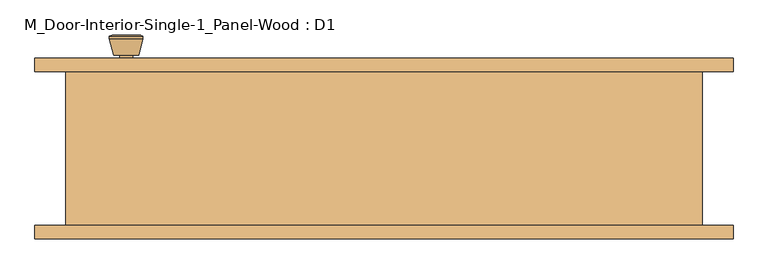
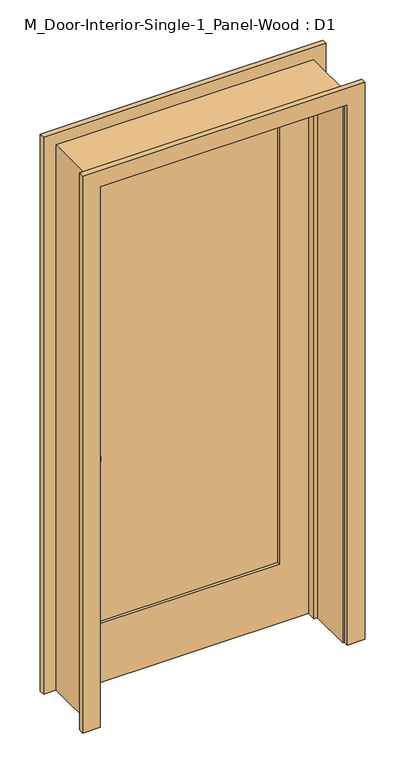
"""IFC4 building model written with IfcOpenShell, lengths in millimetres: door geometry, M_Door-Interior-Single-1_Panel-Wood : D1."""

import ifcopenshell
import ifcopenshell.guid

model = None  # the IFC model being written
_history = None  # IfcOwnerHistory: only IFC2X3 demands one
_inside = {}  # id of a spatial element -> (the spatial element, [elements in it])
_under = {}  # id of a project, library or spatial element -> (it, [spatial elements below it])
_declared = {}  # id of a project -> (the project, [libraries it declares])
_typed = {}  # id of a type object -> (the type object, [elements of that type])
_made_of = {}  # id of a material, layer set ... -> (it, [elements and type objects made of it])


def new_model(schema):
    """Start an empty IFC model of exactly this schema.

    Asked for "IFC4X3", IfcOpenShell would pick the latest addendum, in which some entities
    have other attributes; the version numbers below select the first issue.
    IFC2X3 requires an IfcOwnerHistory on every rooted entity: one is made here for all.
    """
    global model, _history
    if schema == "IFC4X3":
        model = ifcopenshell.file(schema_version=(4, 3, 0, 0))
    else:
        model = ifcopenshell.file(schema=schema)
    _inside.clear()
    _under.clear()
    _declared.clear()
    _typed.clear()
    _made_of.clear()
    _history = None
    if model.schema == "IFC2X3":
        org = make("IfcOrganization", Name="unknown")
        user = make(
            "IfcPersonAndOrganization",
            ThePerson=make("IfcPerson", FamilyName="unknown"),
            TheOrganization=org,
        )
        app = make(
            "IfcApplication",
            ApplicationDeveloper=org,
            Version="unknown",
            ApplicationFullName="unknown",
            ApplicationIdentifier="unknown",
        )
        _history = make(
            "IfcOwnerHistory",
            OwningUser=user,
            OwningApplication=app,
            ChangeAction="ADDED",
            CreationDate=0,
        )
    return model


def make(cls, **values):
    """One entity of the class cls with the attributes given. An attribute that is None is left unset."""
    return model.create_entity(
        cls, **{name: value for name, value in values.items() if value is not None}
    )


def rooted(cls, **values):
    """An entity with a GlobalId (a new one), such as an element, a storey or a relation."""
    return make(cls, GlobalId=ifcopenshell.guid.new(), OwnerHistory=_history, **values)


def si_unit(unit_type, name, prefix=None):
    """IfcSIUnit, for example si_unit("LENGTHUNIT", "METRE", prefix="MILLI")."""
    return make("IfcSIUnit", UnitType=unit_type, Prefix=prefix, Name=name)


def assignment(units):
    """IfcUnitAssignment: the units of a project."""
    return None if units is None else make("IfcUnitAssignment", Units=units)


def point(xyz):
    """IfcCartesianPoint."""
    return None if xyz is None else make("IfcCartesianPoint", Coordinates=xyz)


def direction(xyz):
    """IfcDirection."""
    return None if xyz is None else make("IfcDirection", DirectionRatios=xyz)


def frame(location, z_axis=None, x_axis=None):
    """IfcAxis2Placement3D, a coordinate frame: its origin and axes. An axis left out is left unset."""
    return make(
        "IfcAxis2Placement3D",
        Location=point(location),
        Axis=direction(z_axis),
        RefDirection=direction(x_axis),
    )


def frame_2d(location, x_axis=None):
    """IfcAxis2Placement2D, a coordinate frame in the plane: its origin and x axis."""
    return make(
        "IfcAxis2Placement2D", Location=point(location), RefDirection=direction(x_axis)
    )


def origin():
    """The frame at (0, 0, 0) with its axes left unset."""
    return frame((0.0, 0.0, 0.0))


def place(relative_to, where):
    """IfcLocalPlacement: puts the frame where relative to a parent placement (None: the world)."""
    return make(
        "IfcLocalPlacement", PlacementRelTo=relative_to, RelativePlacement=where
    )


def context(
    kind, dimensions, precision=None, world=None, true_north=None, identifier=None
):
    """IfcGeometricRepresentationContext, for example the 3D "Model" context."""
    return make(
        "IfcGeometricRepresentationContext",
        ContextIdentifier=identifier,
        ContextType=kind,
        CoordinateSpaceDimension=dimensions,
        Precision=precision,
        WorldCoordinateSystem=world,
        TrueNorth=true_north,
    )


def project(units=None, contexts=None):
    """IfcProject with its units and contexts."""
    return rooted(
        "IfcProject",
        Name="project",
        RepresentationContexts=contexts,
        UnitsInContext=assignment(units),
    )


def spatial(cls, under=None, at=None, **own):
    """A site, building, storey or space (cls), placed at a placement, below another one or the project."""
    s = rooted(cls, ObjectPlacement=at, **own)
    if under is not None:
        _under.setdefault(under.id(), (under, []))[1].append(s)
    return s


def polyline(points):
    """IfcPolyline through the points."""
    return make("IfcPolyline", Points=[point(p) for p in points])


def circle_curve(where, radius):
    """IfcCircle in the frame where."""
    return make("IfcCircle", Position=where, Radius=radius)


def trimmed(basis, trim1, trim2, sense, master):
    """IfcTrimmedCurve: the piece of a basis curve between two trims."""
    return make(
        "IfcTrimmedCurve",
        BasisCurve=basis,
        Trim1=trim1,
        Trim2=trim2,
        SenseAgreement=sense,
        MasterRepresentation=master,
    )


def segment(curve, same_sense, transition):
    """IfcCompositeCurveSegment."""
    return make(
        "IfcCompositeCurveSegment",
        Transition=transition,
        SameSense=same_sense,
        ParentCurve=curve,
    )


def composite_curve(segments, self_intersect=None):
    """IfcCompositeCurve: segments joined end to end."""
    return make("IfcCompositeCurve", Segments=segments, SelfIntersect=self_intersect)


def outline(outer, holes=None, kind="AREA"):
    """IfcArbitraryClosedProfileDef: a profile drawn as a closed curve; with holes, ...WithVoids."""
    if holes is None:
        return make("IfcArbitraryClosedProfileDef", ProfileType=kind, OuterCurve=outer)
    return make(
        "IfcArbitraryProfileDefWithVoids",
        ProfileType=kind,
        OuterCurve=outer,
        InnerCurves=holes,
    )


def extrude(swept, where, along, depth):
    """IfcExtrudedAreaSolid: the profile swept, set in the frame where, extruded along a direction by depth."""
    return make(
        "IfcExtrudedAreaSolid",
        SweptArea=swept,
        Position=where,
        ExtrudedDirection=direction(along),
        Depth=depth,
    )


def faces_of(points, faces, orient=None, outer=None):
    """IfcFace entities. A face is a list of loops; a loop is a list of indices into points, from 0.

    orient and outer hold one flag for each loop. By default every Orientation is true, the
    first loop of a face is its IfcFaceOuterBound and the others are IfcFaceBound.
    """
    made = []
    for i, loops in enumerate(faces):
        bounds = []
        for j, loop in enumerate(loops):
            is_outer = j == 0 if outer is None else outer[i][j]
            bounds.append(
                make(
                    "IfcFaceOuterBound" if is_outer else "IfcFaceBound",
                    Bound=make("IfcPolyLoop", Polygon=[points[k] for k in loop]),
                    Orientation=True if orient is None else orient[i][j],
                )
            )
        made.append(make("IfcFace", Bounds=bounds))
    return made


def faceted_brep(points, faces, orient=None, outer=None, voids=None):
    """IfcFacetedBrep: a solid bounded by flat faces; with voids (closed shells), ...WithVoids."""
    shared = [point(p) for p in points]
    hull = make("IfcClosedShell", CfsFaces=faces_of(shared, faces, orient, outer))
    if voids is None:
        return make("IfcFacetedBrep", Outer=hull)
    return make(
        "IfcFacetedBrepWithVoids",
        Outer=hull,
        Voids=[
            make(cls, CfsFaces=faces_of(shared, fs, o, b)) for cls, fs, o, b in voids
        ],
    )


def shape(context_of_items, identifier, shape_type, items):
    """IfcShapeRepresentation: the items that make up one representation, for example the "Body"."""
    return make(
        "IfcShapeRepresentation",
        ContextOfItems=context_of_items,
        RepresentationIdentifier=identifier,
        RepresentationType=shape_type,
        Items=items,
    )


def source(mapping_origin, context_of_items, identifier, shape_type, items):
    """IfcRepresentationMap: a shape defined once, which mapped items show again and again."""
    return make(
        "IfcRepresentationMap",
        MappingOrigin=mapping_origin,
        MappedRepresentation=shape(context_of_items, identifier, shape_type, items),
    )


def transform(
    local_origin,
    x_axis=None,
    y_axis=None,
    z_axis=None,
    scale=None,
    scale2=None,
    scale3=None,
    uniform=True,
):
    """IfcCartesianTransformationOperator3D, or its non-uniform kind. x_axis, y_axis, z_axis: its Axis1, 2, 3."""
    if uniform:
        return make(
            "IfcCartesianTransformationOperator3D",
            Axis1=direction(x_axis),
            Axis2=direction(y_axis),
            LocalOrigin=point(local_origin),
            Scale=scale,
            Axis3=direction(z_axis),
        )
    return make(
        "IfcCartesianTransformationOperator3DnonUniform",
        Axis1=direction(x_axis),
        Axis2=direction(y_axis),
        LocalOrigin=point(local_origin),
        Scale=scale,
        Axis3=direction(z_axis),
        Scale2=scale2,
        Scale3=scale3,
    )


def mapped(mapping_source, mapping_target):
    """IfcMappedItem: shows the shape of a source again, moved by a transform."""
    return make(
        "IfcMappedItem", MappingSource=mapping_source, MappingTarget=mapping_target
    )


def made_of(thing, what):
    """Note that an element or type object is made of a material, layer set ...; save() writes the relation."""
    if what is not None:
        _made_of.setdefault(what.id(), (what, []))[1].append(thing)
    return thing


def element(
    cls,
    number,
    at=None,
    inside=None,
    cuts=None,
    type_object=None,
    material=None,
    context=None,
    identifier="Body",
    shape_type=None,
    held_by="IfcProductDefinitionShape",
    body=None,
    shapes=None,
    **own,
):
    """One element of the class cls, such as IfcWall. Its Tag is "e" and its number.

    at: its placement. inside: the storey or other place that contains it. cuts: it is an
    opening in that element (IfcRelVoidsElement). A single representation is given by context,
    identifier, shape_type and body (its items); several are given by shapes. held_by: the class
    of the entity that holds the representations. save() writes the other relations.
    """
    e = rooted(cls, Tag="e%d" % number, ObjectPlacement=at, **own)
    if body is not None:
        shapes = [shape(context, identifier, shape_type, body)]
    if shapes is not None:
        e.Representation = make(held_by, Representations=shapes)
    if inside is not None:
        _inside.setdefault(inside.id(), (inside, []))[1].append(e)
    if cuts is not None:
        rooted(
            "IfcRelVoidsElement", RelatingBuildingElement=cuts, RelatedOpeningElement=e
        )
    if type_object is not None:
        _typed.setdefault(type_object.id(), (type_object, []))[1].append(e)
    return made_of(e, material)


def aggregate(whole, parts):
    """IfcRelAggregates: a whole, such as a stair, and the parts it consists of."""
    return rooted("IfcRelAggregates", RelatingObject=whole, RelatedObjects=parts)


def save(model, path):
    """Write the relations noted so far, then the file.

    IfcRelAggregates (storeys below a building ...), IfcRelContainedInSpatialStructure (elements
    in a storey), IfcRelDefinesByType, IfcRelAssociatesMaterial and IfcRelDeclares: one each for
    every whole, place, type object, material and project.
    """
    for whole, parts in _under.values():
        aggregate(whole, parts)
    for where, things in _inside.values():
        rooted(
            "IfcRelContainedInSpatialStructure",
            RelatedElements=things,
            RelatingStructure=where,
        )
    for kind, things in _typed.values():
        rooted("IfcRelDefinesByType", RelatedObjects=things, RelatingType=kind)
    for what, things in _made_of.values():
        rooted("IfcRelAssociatesMaterial", RelatedObjects=things, RelatingMaterial=what)
    for by, libraries in _declared.values():
        rooted("IfcRelDeclares", RelatingContext=by, RelatedDefinitions=libraries)
    model.write(path)


def plane_surface(at):
    """IfcPlane: the flat surface through the origin of the frame at, square to its z axis."""
    return make("IfcPlane", Position=at)


def cylinder_surface(at, radius):
    """IfcCylindricalSurface: all points at the distance radius from the z axis of the frame at."""
    return make("IfcCylindricalSurface", Position=at, Radius=radius)


def revolved_surface(curve, axis_point, axis_direction):
    """IfcSurfaceOfRevolution: the curve turned about the line through axis_point along axis_direction."""
    return make(
        "IfcSurfaceOfRevolution",
        SweptCurve=make("IfcArbitraryOpenProfileDef", ProfileType="CURVE", Curve=curve),
        AxisPosition=make("IfcAxis1Placement", Location=point(axis_point), Axis=direction(axis_direction)),
    )


def advanced_brep(points, edges, surfaces, faces):
    """IfcAdvancedBrep: a solid bounded by faces that lie on surfaces and meet in shared edges.

    An edge is (start, end): straight between two places in points (the first is 0);
    or (start, end, curve); or (start, end, curve, False) where it runs against its curve.
    A face is (place in surfaces, loops), or (place, loops, False) where it looks against
    its surface's normal. A loop lists edges by number (the first is 1), with a minus sign
    where the edge is run from its end to its start. The first loop is the outer one.
    """
    corners = [point(p) for p in points]
    vertices = [make("IfcVertexPoint", VertexGeometry=c) for c in corners]
    made = []
    for start, end, *more in edges:
        made.append(
            make(
                "IfcEdgeCurve",
                EdgeStart=vertices[start],
                EdgeEnd=vertices[end],
                EdgeGeometry=more[0] if more else make("IfcPolyline", Points=[corners[start], corners[end]]),
                SameSense=more[1] if len(more) > 1 else True,
            )
        )
    hull = []
    for where, loops, *sense in faces:
        bounds = []
        for j, loop in enumerate(loops):
            ring = [make("IfcOrientedEdge", EdgeElement=made[abs(k) - 1], Orientation=k > 0) for k in loop]
            bounds.append(
                make(
                    "IfcFaceOuterBound" if j == 0 else "IfcFaceBound",
                    Bound=make("IfcEdgeLoop", EdgeList=ring),
                    Orientation=True,
                )
            )
        hull.append(make("IfcAdvancedFace", Bounds=bounds, FaceSurface=surfaces[where], SameSense=sense[0] if sense else True))
    return make("IfcAdvancedBrep", Outer=make("IfcClosedShell", CfsFaces=hull))


def m_door_interior_single_1_panel_wood_d1_706e19ec(model_context):
    return source(origin(), model_context, "Body", "SolidModel", [
        advanced_brep(
        [(-385.0, 70.825, 914.4), (-375.0, 70.825, 914.4), (-395.0, 70.825, 914.4), (-364.5241324, 21.825, 914.4), (-385.0, 21.825, 914.4), (-405.4758676, 21.825, 914.4), (-360.0, 23.6528681, 914.4), (-410.0, 23.6528681, 914.4), (-360.0, 27.1165463, 914.4), (-410.0, 27.1165463, 914.4), (-366.363764, 51.825, 914.4), (-403.636236, 51.825, 914.4), (-375.0, 51.825, 914.4), (-395.0, 51.825, 914.4)],
        [
            (0, 1),
            (1, 2, circle_curve(frame((-385.0, 70.825, 914.4), z_axis=(0.0, 1.0, 0.0), x_axis=(-1.0, 0.0, 0.0)), 10.0)),
            (2, 0),
            (2, 1, circle_curve(frame((-385.0, 70.825, 914.4), z_axis=(0.0, 1.0, 0.0), x_axis=(-1.0, 0.0, 0.0)), 10.0)),
            (3, 4),
            (4, 5),
            (5, 3, circle_curve(frame((-385.0, 21.825, 914.4), z_axis=(0.0, -1.0, 0.0), x_axis=(-1.0, 0.0, 0.0)), 20.4758676)),
            (3, 5, circle_curve(frame((-385.0, 21.825, 914.4), z_axis=(0.0, -1.0, 0.0), x_axis=(-1.0, 0.0, 0.0)), 20.4758676)),
            (6, 3),
            (5, 7),
            (7, 6, circle_curve(frame((-385.0, 23.6528681, 914.4), z_axis=(0.0, -1.0, 0.0), x_axis=(-1.0, 0.0, 0.0)), 25.0)),
            (6, 7, circle_curve(frame((-385.0, 23.6528681, 914.4), z_axis=(0.0, -1.0, 0.0), x_axis=(-1.0, 0.0, 0.0)), 25.0)),
            (8, 6),
            (7, 9),
            (9, 8, circle_curve(frame((-385.0, 27.1165463, 914.4), z_axis=(0.0, -1.0, 0.0), x_axis=(-1.0, 0.0, 0.0)), 25.0)),
            (8, 9, circle_curve(frame((-385.0, 27.1165463, 914.4), z_axis=(0.0, -1.0, 0.0), x_axis=(-1.0, 0.0, 0.0)), 25.0)),
            (10, 8),
            (9, 11),
            (11, 10, circle_curve(frame((-385.0, 51.825, 914.4), z_axis=(0.0, -1.0, 0.0), x_axis=(-1.0, 0.0, 0.0)), 18.636236)),
            (10, 11, circle_curve(frame((-385.0, 51.825, 914.4), z_axis=(0.0, -1.0, 0.0), x_axis=(-1.0, 0.0, 0.0)), 18.636236)),
            (12, 10),
            (11, 13),
            (13, 12, circle_curve(frame((-385.0, 51.825, 914.4), z_axis=(0.0, -1.0, 0.0), x_axis=(-1.0, 0.0, 0.0)), 10.0)),
            (12, 13, circle_curve(frame((-385.0, 51.825, 914.4), z_axis=(0.0, -1.0, 0.0), x_axis=(-1.0, 0.0, 0.0)), 10.0)),
            (1, 12),
            (13, 2),
        ],
        [
            plane_surface(frame((-385.0, 70.825, 914.4), z_axis=(0.0, 1.0, 0.0), x_axis=(-1.0, 0.0, 0.0))),
            plane_surface(frame((-385.0, 21.825, 914.4), z_axis=(0.0, -1.0, 0.0), x_axis=(-1.0, 0.0, 0.0))),
            revolved_surface(polyline([(-405.4758676, 21.825, 914.4), (-410.0, 23.6528681, 914.4)]), (-385.0, 70.825, 914.4), (0.0, 1.0, 0.0)),
            cylinder_surface(frame((-385.0, 70.825, 914.4), z_axis=(0.0, 1.0, 0.0), x_axis=(-1.0, 0.0, 0.0)), 25.0),
            revolved_surface(polyline([(-410.0, 27.1165463, 914.4), (-403.636236, 51.825, 914.4)]), (-385.0, 70.825, 914.4), (0.0, 1.0, 0.0)),
            plane_surface(frame((-385.0, 51.825, 914.4), z_axis=(0.0, 1.0, 0.0), x_axis=(-1.0, 0.0, 0.0))),
            cylinder_surface(frame((-385.0, 70.825, 914.4), z_axis=(0.0, 1.0, 0.0), x_axis=(-1.0, 0.0, 0.0)), 10.0),
        ],
        [
            (0, [[1, 2, 3]]),
            (0, [[-3, 4, -1]]),
            (1, [[5, 6, 7]]),
            (1, [[-6, -5, 8]]),
            (2, [[9, -7, 10, 11]]),
            (2, [[-10, -8, -9, 12]]),
            (3, [[13, -11, 14, 15]]),
            (3, [[-14, -12, -13, 16]]),
            (4, [[17, -15, 18, 19]]),
            (4, [[-18, -16, -17, 20]]),
            (5, [[21, -19, 22, 23]]),
            (5, [[-22, -20, -21, 24]]),
            (6, [[25, -23, 26, -2]]),
            (6, [[-26, -24, -25, -4]]),
        ],
    ),
        extrude(outline(composite_curve([segment(trimmed(circle_curve(frame_2d((914.4, -385.0)), 30.0), [point((914.4, -415.0))], [point((914.4, -355.0))], False, "CARTESIAN"), True, "CONTINUOUS"), segment(trimmed(circle_curve(frame_2d((914.4, -385.0)), 30.0), [point((914.4, -355.0))], [point((914.4, -415.0))], False, "CARTESIAN"), True, "CONTINUOUS")], self_intersect=False)), frame((0.0, 70.825, 0.0), z_axis=(0.0, 1.0, 0.0), x_axis=(0.0, 0.0, 1.0)), (0.0, 0.0, 1.0), 6.0),
        advanced_brep(
        [(-385.0, 117.825, 914.4), (-395.0, 117.825, 914.4), (-375.0, 117.825, 914.4), (-364.5241324, 166.825, 914.4), (-405.4758676, 166.825, 914.4), (-385.0, 166.825, 914.4), (-360.0, 164.9971319, 914.4), (-410.0, 164.9971319, 914.4), (-360.0, 161.5334537, 914.4), (-410.0, 161.5334537, 914.4), (-366.363764, 136.825, 914.4), (-403.636236, 136.825, 914.4), (-375.0, 136.825, 914.4), (-395.0, 136.825, 914.4)],
        [
            (0, 1),
            (1, 2, circle_curve(frame((-385.0, 117.825, 914.4), z_axis=(0.0, -1.0, 0.0), x_axis=(-1.0, 0.0, 0.0)), 10.0)),
            (2, 0),
            (2, 1, circle_curve(frame((-385.0, 117.825, 914.4), z_axis=(0.0, -1.0, 0.0), x_axis=(-1.0, 0.0, 0.0)), 10.0)),
            (3, 4, circle_curve(frame((-385.0, 166.825, 914.4), z_axis=(0.0, 1.0, 0.0), x_axis=(-1.0, 0.0, 0.0)), 20.4758676)),
            (4, 5),
            (5, 3),
            (4, 3, circle_curve(frame((-385.0, 166.825, 914.4), z_axis=(0.0, 1.0, 0.0), x_axis=(-1.0, 0.0, 0.0)), 20.4758676)),
            (6, 7, circle_curve(frame((-385.0, 164.9971319, 914.4), z_axis=(0.0, 1.0, 0.0), x_axis=(-1.0, 0.0, 0.0)), 25.0)),
            (7, 4),
            (3, 6),
            (7, 6, circle_curve(frame((-385.0, 164.9971319, 914.4), z_axis=(0.0, 1.0, 0.0), x_axis=(-1.0, 0.0, 0.0)), 25.0)),
            (8, 9, circle_curve(frame((-385.0, 161.5334537, 914.4), z_axis=(0.0, 1.0, 0.0), x_axis=(-1.0, 0.0, 0.0)), 25.0)),
            (9, 7),
            (6, 8),
            (9, 8, circle_curve(frame((-385.0, 161.5334537, 914.4), z_axis=(0.0, 1.0, 0.0), x_axis=(-1.0, 0.0, 0.0)), 25.0)),
            (10, 11, circle_curve(frame((-385.0, 136.825, 914.4), z_axis=(0.0, 1.0, 0.0), x_axis=(-1.0, 0.0, 0.0)), 18.636236)),
            (11, 9),
            (8, 10),
            (11, 10, circle_curve(frame((-385.0, 136.825, 914.4), z_axis=(0.0, 1.0, 0.0), x_axis=(-1.0, 0.0, 0.0)), 18.636236)),
            (12, 13, circle_curve(frame((-385.0, 136.825, 914.4), z_axis=(0.0, 1.0, 0.0), x_axis=(-1.0, 0.0, 0.0)), 10.0)),
            (13, 11),
            (10, 12),
            (13, 12, circle_curve(frame((-385.0, 136.825, 914.4), z_axis=(0.0, 1.0, 0.0), x_axis=(-1.0, 0.0, 0.0)), 10.0)),
            (1, 13),
            (12, 2),
        ],
        [
            plane_surface(frame((-385.0, 117.825, 914.4), z_axis=(0.0, -1.0, 0.0), x_axis=(-1.0, 0.0, 0.0))),
            plane_surface(frame((-385.0, 166.825, 914.4), z_axis=(0.0, 1.0, 0.0), x_axis=(-1.0, 0.0, 0.0))),
            revolved_surface(polyline([(-405.4758676, 166.825, 914.4), (-410.0, 164.9971319, 914.4)]), (-385.0, 117.825, 914.4), (0.0, -1.0, 0.0)),
            cylinder_surface(frame((-385.0, 117.825, 914.4), z_axis=(0.0, -1.0, 0.0), x_axis=(-1.0, 0.0, 0.0)), 25.0),
            revolved_surface(polyline([(-410.0, 161.5334537, 914.4), (-403.636236, 136.825, 914.4)]), (-385.0, 117.825, 914.4), (0.0, -1.0, 0.0)),
            plane_surface(frame((-385.0, 136.825, 914.4), z_axis=(0.0, -1.0, 0.0), x_axis=(-1.0, 0.0, 0.0))),
            cylinder_surface(frame((-385.0, 117.825, 914.4), z_axis=(0.0, -1.0, 0.0), x_axis=(-1.0, 0.0, 0.0)), 10.0),
        ],
        [
            (0, [[1, 2, 3]]),
            (0, [[-3, 4, -1]]),
            (1, [[5, 6, 7]]),
            (1, [[8, -7, -6]]),
            (2, [[9, 10, -5, 11]]),
            (2, [[12, -11, -8, -10]]),
            (3, [[13, 14, -9, 15]]),
            (3, [[16, -15, -12, -14]]),
            (4, [[17, 18, -13, 19]]),
            (4, [[20, -19, -16, -18]]),
            (5, [[21, 22, -17, 23]]),
            (5, [[24, -23, -20, -22]]),
            (6, [[-2, 25, -21, 26]]),
            (6, [[-4, -26, -24, -25]]),
        ],
    ),
        extrude(outline(composite_curve([segment(trimmed(circle_curve(frame_2d((914.4, -385.0)), 30.0), [point((914.4, -415.0))], [point((914.4, -355.0))], False, "CARTESIAN"), True, "CONTINUOUS"), segment(trimmed(circle_curve(frame_2d((914.4, -385.0)), 30.0), [point((914.4, -355.0))], [point((914.4, -415.0))], False, "CARTESIAN"), True, "CONTINUOUS")], self_intersect=False)), frame((0.0, 111.825, 0.0), z_axis=(0.0, 1.0, 0.0), x_axis=(0.0, 0.0, 1.0)), (0.0, 0.0, 1.0), 6.0),
        extrude(outline(polyline([(330.0, 88.4916667), (-330.0, 88.4916667), (-330.0, 100.1583333), (330.0, 100.1583333), (330.0, 88.4916667)])), frame((0.0, 0.0, 230.0), z_axis=(0.0, 0.0, 1.0), x_axis=(1.0, 0.0, 0.0)), (0.0, 0.0, 1.0), 1750.0),
        extrude(outline(polyline([(2100.0, -450.0), (0.0, -450.0), (0.0, 450.0), (2100.0, 450.0), (2100.0, -450.0)]), holes=[polyline([(1980.0, -330.0), (1980.0, 330.0), (230.0, 330.0), (230.0, -330.0), (1980.0, -330.0)])]), frame((0.0, 76.825, 0.0), z_axis=(0.0, 1.0, 0.0), x_axis=(0.0, 0.0, 1.0)), (0.0, 0.0, 1.0), 35.0),
        faceted_brep([(475.0, 111.825, 0.0), (475.0, -118.175, 0.0), (450.0, -118.175, 0.0), (450.0, 41.9, 0.0), (437.3, 41.9, 0.0), (437.3, 76.825, 0.0), (450.0, 76.825, 0.0), (450.0, 111.825, 0.0), (475.0, 111.825, 2125.0), (475.0, -118.175, 2125.0), (-475.0, -118.175, 2125.0), (-475.0, -118.175, 0.0), (-450.0, -118.175, 0.0), (-450.0, -118.175, 2100.0), (450.0, -118.175, 2100.0), (450.0, 41.9, 2100.0), (-450.0, 41.9, 2100.0), (-450.0, 41.9, 0.0), (-437.3, 41.9, 0.0), (-437.3, 41.9, 2087.3), (437.3, 41.9, 2087.3), (437.3, 76.825, 2087.3), (-437.3, 76.825, 2087.3), (-437.3, 76.825, 0.0), (-450.0, 76.825, 0.0), (-450.0, 76.825, 2100.0), (450.0, 76.825, 2100.0), (450.0, 111.825, 2100.0), (-450.0, 111.825, 2100.0), (-450.0, 111.825, 0.0), (-475.0, 111.825, 0.0), (-475.0, 111.825, 2125.0)], [[[0, 1, 2, 3, 4, 5, 6, 7]], [[1, 0, 8, 9]], [[2, 1, 9, 10, 11, 12, 13, 14]], [[3, 2, 14, 15]], [[4, 3, 15, 16, 17, 18, 19, 20]], [[5, 4, 20, 21]], [[6, 5, 21, 22, 23, 24, 25, 26]], [[7, 6, 26, 27]], [[0, 7, 27, 28, 29, 30, 31, 8]], [[9, 8, 31, 10]], [[15, 14, 13, 16]], [[21, 20, 19, 22]], [[27, 26, 25, 28]], [[30, 29, 24, 23, 18, 17, 12, 11]], [[10, 31, 30, 11]], [[16, 13, 12, 17]], [[22, 19, 18, 23]], [[28, 25, 24, 29]]]),
        extrude(outline(polyline([(0.0, 456.35), (0.0, 521.35), (2171.35, 521.35), (2171.35, -521.35), (0.0, -521.35), (0.0, -456.35), (2106.35, -456.35), (2106.35, 456.35), (0.0, 456.35)])), frame((0.0, -138.175, 0.0), z_axis=(0.0, 1.0, 0.0), x_axis=(0.0, 0.0, 1.0)), (0.0, 0.0, 1.0), 20.0),
        extrude(outline(polyline([(0.0, 456.35), (0.0, 521.35), (2171.35, 521.35), (2171.35, -521.35), (0.0, -521.35), (0.0, -456.35), (2106.35, -456.35), (2106.35, 456.35), (0.0, 456.35)])), frame((0.0, 111.825, 0.0), z_axis=(0.0, 1.0, 0.0), x_axis=(0.0, 0.0, 1.0)), (0.0, 0.0, 1.0), 20.0),
    ])


if __name__ == "__main__":
    model = new_model("IFC4")
    model_context = context("Model", 3, world=origin())
    ifc_project = project(units=[si_unit("LENGTHUNIT", "METRE", prefix="MILLI")], contexts=[model_context])
    site = spatial("IfcSite", under=ifc_project)
    building = spatial("IfcBuilding", under=site)
    placement = place(None, origin())
    m_door_interior_single_1_panel_wood_d1_shape = m_door_interior_single_1_panel_wood_d1_706e19ec(model_context)
    element("IfcDoor", 1, ObjectType="M_Door-Interior-Single-1_Panel-Wood : D1", at=placement, inside=building, context=model_context, shape_type="MappedRepresentation", body=[
        mapped(m_door_interior_single_1_panel_wood_d1_shape, transform((0.0, 0.0, 0.0), x_axis=(1.0, 0.0, 0.0), y_axis=(0.0, 1.0, 0.0), z_axis=(0.0, 0.0, 1.0))),
    ])
    save(model, "model.ifc")

# Revit data of these elements
# Type "M_Door-Interior-Single-1_Panel-Wood : D1"
#   Type Mark = "49"
#   Assembly Code = "C1020300"
#   Analytic Construction = "Wooden"
#   Top Rail = 12 cm
#   Thickness = 3.5 cm
#   Thermal Resistance (R) = 0.455703 (m²·K)/W
#   Swing Angle [instance default] = 90.00°
#   Stiles = 12 cm
#   Rough Width = 95 cm
#   Rough Height = 212.5 cm
#   Height = 210 cm
#   Width = 90 cm
#   Heat Transfer Coefficient (U) = 2.19465 W/(m²·K)
#   Bottom Rail = 23 cm
#   Trim Material = Cherry
#   Panel Material = Cherry
#   Frame Material = Cherry
#   Door Handle Material = Aluminum
#   Visual Light Transmittance = 0
#   Solar Heat Gain Coefficient = 0
#   Wall Closure = (empty or 0)
#   Function = (empty or 0)
# Element 1 (IfcDoor, "M_Door-Interior-Single-1_Panel-Wood : D1")
#   Materials on its faces: "Cherry", "Aluminum"
# Materials
#   "Cherry": class "Wood", colour RGB 226 177 128, transparency 0, Description = "Prunus Serotina", Cost = 0
#   "Aluminum": class "Metal", colour RGB 247 247 247, transparency 0, Description = "Aluminum 6061", Cost = 0
